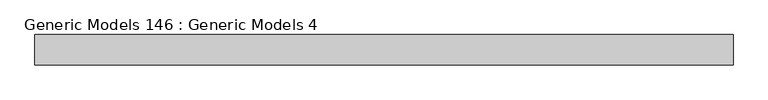
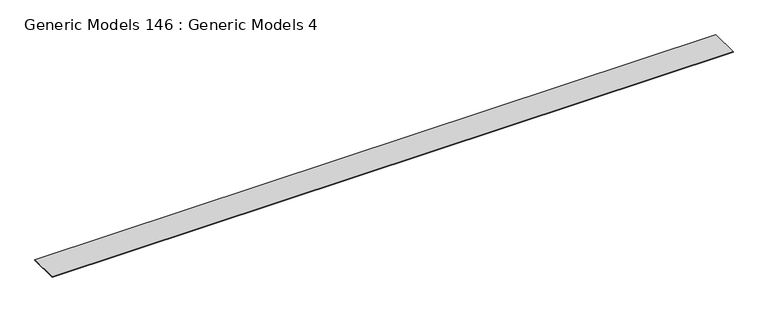
"""IFC4 building model written with IfcOpenShell, lengths in millimetres: proxy geometry, Generic Models 146 : Generic Models 4."""

from ifc_helpers import new_model, si_unit, frame, origin, place, context, project, spatial, polyline, outline, extrude, source, transform, mapped, element, save


def generic_models_146_generic_models_4_285cb4c9(model_context):
    return source(origin(), model_context, "Body", "SweptSolid", [
        extrude(outline(polyline([(20644.6159513, 7212.6867903), (20644.6159513, 7761.1754549), (33192.2159513, 7761.1754549), (33192.2159513, 7212.6867903), (20644.6159513, 7212.6867903)])), frame((0.0, 0.0, 124028.7951265), z_axis=(0.0, 0.0, 1.0), x_axis=(1.0, 0.0, 0.0)), (0.0, 0.0, 1.0), 1.5875),
    ])


if __name__ == "__main__":
    model = new_model("IFC4")
    model_context = context("Model", 3, world=origin())
    ifc_project = project(units=[si_unit("LENGTHUNIT", "METRE", prefix="MILLI")], contexts=[model_context])
    site = spatial("IfcSite", under=ifc_project)
    building = spatial("IfcBuilding", under=site)
    placement = place(None, origin())
    generic_models_146_generic_models_4_shape = generic_models_146_generic_models_4_285cb4c9(model_context)
    element("IfcBuildingElementProxy", 1, Name="Generic Models 146 : Generic Models 4", ObjectType="Generic Models 146 : Generic Models 4", at=placement, inside=building, context=model_context, shape_type="MappedRepresentation", body=[
        mapped(generic_models_146_generic_models_4_shape, transform((0.0, 0.0, 0.0), x_axis=(1.0, 0.0, 0.0), y_axis=(0.0, 1.0, 0.0), z_axis=(0.0, 0.0, 1.0))),
    ])
    save(model, "model.ifc")

# Revit data of these elements
# Element 1 (IfcBuildingElementProxy, "Generic Models 146 : Generic Models 4")
#   Materials on its faces: "_6 MIL VAPOR BARRIER"
# Materials
#   "_6 MIL VAPOR BARRIER": class "Generic", colour RGB 67 154 161, transparency 0, Cost = 0
